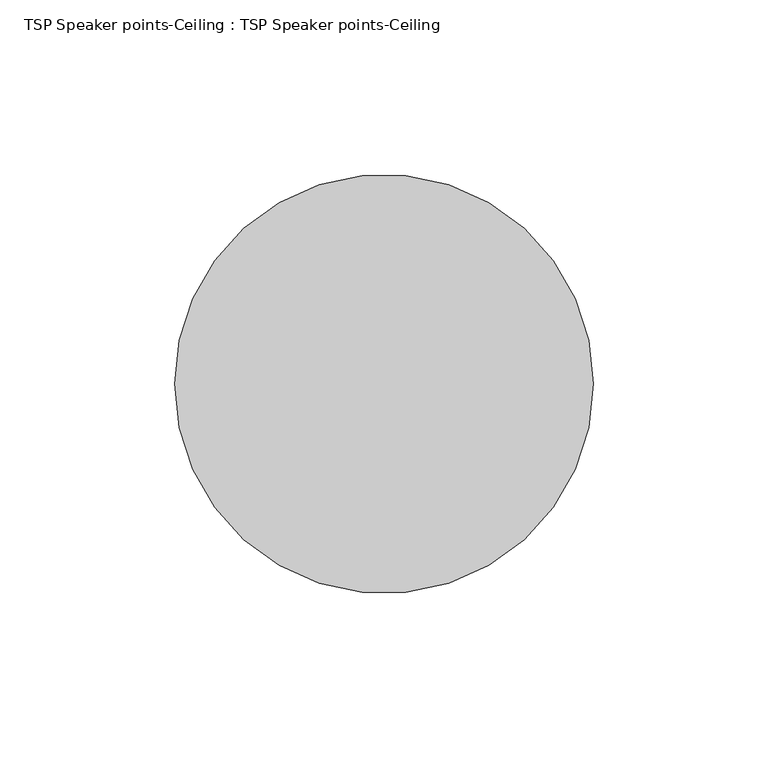
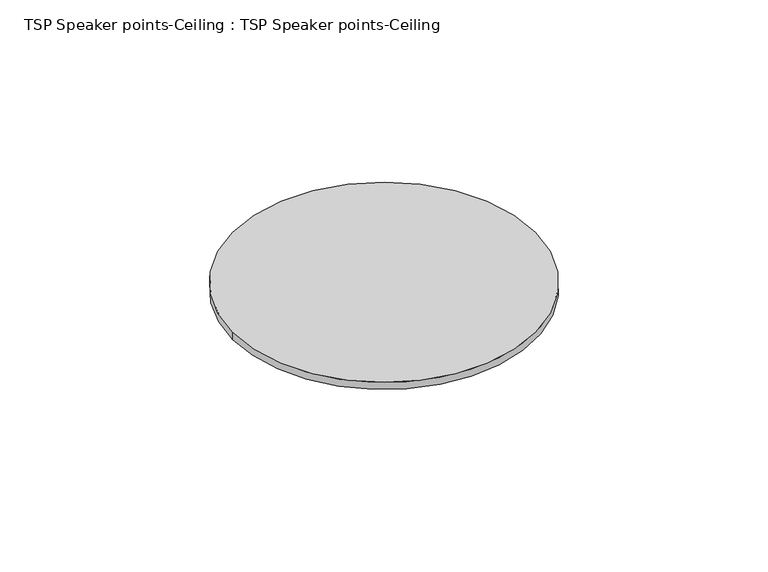
"""IFC4 building model written with IfcOpenShell, lengths in millimetres: proxy geometry, TSP Speaker points-Ceiling : TSP Speaker points-Ceiling."""

from ifc_helpers import new_model, si_unit, point, frame_2d, origin, origin_with_axes, place, context, project, spatial, circle_curve, trimmed, segment, composite_curve, outline, extrude, source, transform, mapped, element, save


def tsp_speaker_points_ceiling_tsp_speaker_points_ceiling_6d6b0419(model_context):
    return source(origin(), model_context, "Body", "SweptSolid", [
        extrude(outline(composite_curve([segment(trimmed(circle_curve(frame_2d((-74.5076114, 0.0)), 60.0), [point((-134.5076114, 0.0))], [point((-14.5076114, 0.0))], False, "CARTESIAN"), True, "CONTINUOUS"), segment(trimmed(circle_curve(frame_2d((-74.5076114, 0.0)), 60.0), [point((-14.5076114, 0.0))], [point((-134.5076114, 0.0))], False, "CARTESIAN"), True, "CONTINUOUS")], self_intersect=False)), origin_with_axes(), (0.0, 0.0, 1.0), 3.0),
    ])


if __name__ == "__main__":
    model = new_model("IFC4")
    model_context = context("Model", 3, world=origin())
    ifc_project = project(units=[si_unit("LENGTHUNIT", "METRE", prefix="MILLI")], contexts=[model_context])
    site = spatial("IfcSite", under=ifc_project)
    building = spatial("IfcBuilding", under=site)
    placement = place(None, origin())
    tsp_speaker_points_ceiling_tsp_speaker_points_ceiling_shape = tsp_speaker_points_ceiling_tsp_speaker_points_ceiling_6d6b0419(model_context)
    element("IfcBuildingElementProxy", 1, Name="TSP Speaker points-Ceiling : TSP Speaker points-Ceiling", ObjectType="TSP Speaker points-Ceiling : TSP Speaker points-Ceiling", at=placement, inside=building, context=model_context, shape_type="MappedRepresentation", body=[
        mapped(tsp_speaker_points_ceiling_tsp_speaker_points_ceiling_shape, transform((0.0, 0.0, 0.0), x_axis=(1.0, 0.0, 0.0), y_axis=(0.0, 1.0, 0.0), z_axis=(0.0, 0.0, 1.0))),
    ])
    save(model, "model.ifc")

# Revit data of these elements
# Type "TSP Speaker points-Ceiling : TSP Speaker points-Ceiling"
#   Model = "TSP_ELECSPEAKCEIL"
#   Default Elevation = 0
# Element 1 (IfcBuildingElementProxy, "TSP Speaker points-Ceiling : TSP Speaker points-Ceiling")
#   Materials on its faces: "Cellulose Fill"
# Materials
#   "Cellulose Fill": class "Generic", colour RGB 0 0 0, transparency 0, Description = "Cellulose loose fill", Cost = 0
